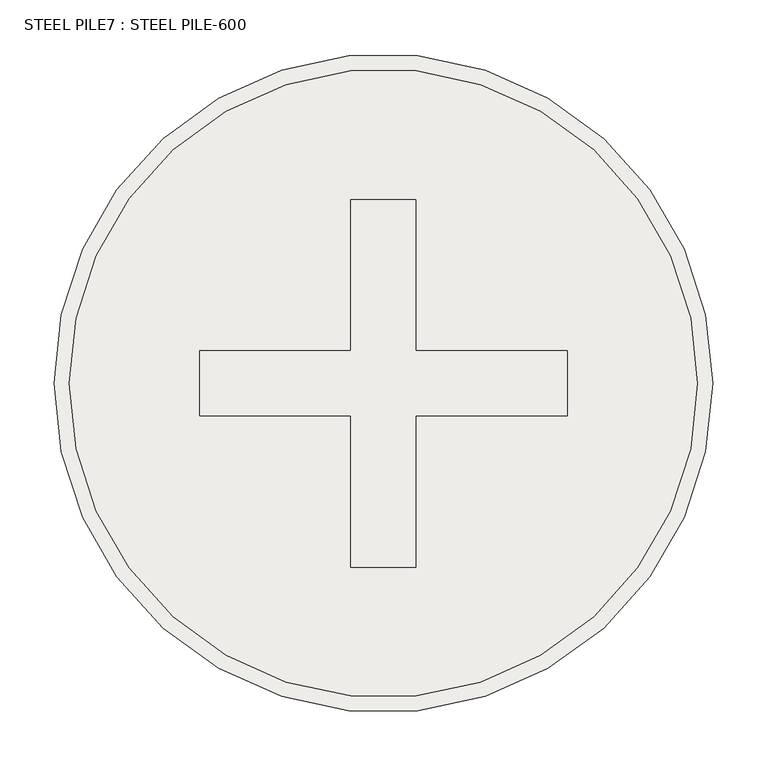
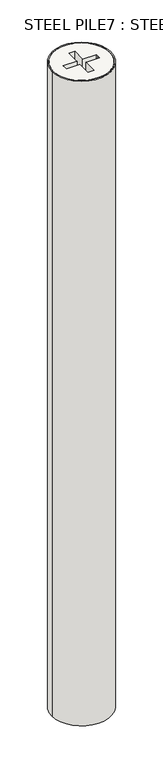
"""IFC4 building model written with IfcOpenShell, lengths in millimetres: slab geometry, STEEL PILE7 : STEEL PILE-600."""

from ifc_helpers import new_model, si_unit, point, frame, frame_2d, origin, place, context, project, spatial, circle_curve, trimmed, segment, composite_curve, outline, extrude, source, transform, mapped, element, save
from ifc_brep_helpers import plane_surface, cylinder_surface, advanced_brep


def steel_pile7_steel_pile_600_8fff8169(model_context):
    return source(origin(), model_context, "Body", "SolidModel", [
        advanced_brep(
        [(14709.5, 22499.5208589, 150.0), (15290.5, 22499.5208589, 150.0), (14970.0, 22469.5208589, 150.0), (14830.0, 22469.5208589, 150.0), (14830.0, 22499.5208589, 150.0), (14830.0, 22529.5208589, 150.0), (14970.0, 22529.5208589, 150.0), (14970.0, 22669.5208589, 150.0), (15030.0, 22669.5208589, 150.0), (15030.0, 22529.5208589, 150.0), (15170.0, 22529.5208589, 150.0), (15170.0, 22499.5208589, 150.0), (15170.0, 22469.5208589, 150.0), (15030.0, 22469.5208589, 150.0), (15030.0, 22329.5208589, 150.0), (14970.0, 22329.5208589, 150.0), (14709.5, 22499.5208589, -1850.0), (15290.5, 22499.5208589, -1850.0), (14830.0, 22469.5208589, -160.0), (14970.0, 22469.5208589, -160.0), (14970.0, 22329.5208589, -160.0), (15030.0, 22329.5208589, -160.0), (15030.0, 22469.5208589, -160.0), (15170.0, 22469.5208589, -160.0), (15170.0, 22499.5208589, -160.0), (15170.0, 22529.5208589, -160.0), (15030.0, 22529.5208589, -160.0), (15030.0, 22669.5208589, -160.0), (14970.0, 22669.5208589, -160.0), (14970.0, 22529.5208589, -160.0), (14830.0, 22529.5208589, -160.0), (14830.0, 22499.5208589, -160.0)],
        [
            (0, 1, circle_curve(frame((15000.0, 22499.5208589, 150.0), z_axis=(0.0, 0.0, 1.0), x_axis=(1.0, 0.0, 0.0)), 290.5)),
            (1, 0, circle_curve(frame((15000.0, 22499.5208589, 150.0), z_axis=(0.0, 0.0, 1.0), x_axis=(1.0, 0.0, 0.0)), 290.5)),
            (2, 3),
            (3, 4),
            (4, 5),
            (5, 6),
            (6, 7),
            (7, 8),
            (8, 9),
            (9, 10),
            (10, 11),
            (11, 12),
            (12, 13),
            (13, 14),
            (14, 15),
            (15, 2),
            (16, 17, circle_curve(frame((15000.0, 22499.5208589, -1850.0), z_axis=(0.0, 0.0, -1.0), x_axis=(1.0, 0.0, 0.0)), 290.5)),
            (17, 16, circle_curve(frame((15000.0, 22499.5208589, -1850.0), z_axis=(0.0, 0.0, -1.0), x_axis=(1.0, 0.0, 0.0)), 290.5)),
            (0, 16),
            (17, 1),
            (18, 19),
            (19, 20),
            (20, 21),
            (21, 22),
            (22, 23),
            (23, 24),
            (24, 25),
            (25, 26),
            (26, 27),
            (27, 28),
            (28, 29),
            (29, 30),
            (30, 31),
            (31, 18),
            (18, 3),
            (2, 19),
            (15, 20),
            (14, 21),
            (13, 22),
            (12, 23),
            (11, 24),
            (10, 25),
            (9, 26),
            (8, 27),
            (7, 28),
            (6, 29),
            (5, 30),
            (4, 31),
        ],
        [
            plane_surface(frame((15290.5, 22499.5208589, 150.0), z_axis=(0.0, 0.0, 1.0), x_axis=(0.0, 1.0, 0.0))),
            plane_surface(frame((15290.5, 22499.5208589, -1850.0), z_axis=(0.0, 0.0, -1.0), x_axis=(0.0, -1.0, 0.0))),
            cylinder_surface(frame((15000.0, 22499.5208589, -1850.0), z_axis=(0.0, 0.0, 1.0), x_axis=(1.0, 0.0, 0.0)), 290.5),
            plane_surface(frame((14830.0, 22469.5208589, -160.0), z_axis=(0.0, 0.0, 1.0), x_axis=(-1.0, 0.0, 0.0))),
            plane_surface(frame((14830.0, 22469.5208589, 160.0), z_axis=(0.0, 1.0, 0.0), x_axis=(0.0, 0.0, -1.0))),
            plane_surface(frame((14970.0, 22469.5208589, 160.0), z_axis=(1.0, 0.0, 0.0), x_axis=(0.0, 0.0, -1.0))),
            plane_surface(frame((14970.0, 22329.5208589, 160.0), z_axis=(0.0, 1.0, 0.0), x_axis=(0.0, 0.0, -1.0))),
            plane_surface(frame((15030.0, 22329.5208589, 160.0), z_axis=(-1.0, 0.0, 0.0), x_axis=(0.0, 0.0, -1.0))),
            plane_surface(frame((15030.0, 22469.5208589, 160.0), z_axis=(0.0, 1.0, 0.0), x_axis=(0.0, 0.0, -1.0))),
            plane_surface(frame((15170.0, 22469.5208589, 160.0), z_axis=(-1.0, 0.0, 0.0), x_axis=(0.0, 0.0, -1.0))),
            plane_surface(frame((15170.0, 22499.5208589, 160.0), z_axis=(-1.0, 0.0, 0.0), x_axis=(0.0, 0.0, -1.0))),
            plane_surface(frame((15170.0, 22529.5208589, 160.0), z_axis=(0.0, -1.0, 0.0), x_axis=(0.0, 0.0, -1.0))),
            plane_surface(frame((15030.0, 22529.5208589, 160.0), z_axis=(-1.0, 0.0, 0.0), x_axis=(0.0, 0.0, -1.0))),
            plane_surface(frame((15030.0, 22669.5208589, 160.0), z_axis=(0.0, -1.0, 0.0), x_axis=(0.0, 0.0, -1.0))),
            plane_surface(frame((14970.0, 22669.5208589, 160.0), z_axis=(1.0, 0.0, 0.0), x_axis=(0.0, 0.0, -1.0))),
            plane_surface(frame((14970.0, 22529.5208589, 160.0), z_axis=(0.0, -1.0, 0.0), x_axis=(0.0, 0.0, -1.0))),
            plane_surface(frame((14830.0, 22529.5208589, 160.0), z_axis=(1.0, 0.0, 0.0), x_axis=(0.0, 0.0, -1.0))),
            plane_surface(frame((14830.0, 22499.5208589, 160.0), z_axis=(1.0, 0.0, 0.0), x_axis=(0.0, 0.0, -1.0))),
        ],
        [
            (0, [[1, 2], [3, 4, 5, 6, 7, 8, 9, 10, 11, 12, 13, 14, 15, 16]]),
            (1, [[17, 18]]),
            (2, [[-1, 19, -18, 20]]),
            (2, [[-2, -20, -17, -19]]),
            (3, [[21, 22, 23, 24, 25, 26, 27, 28, 29, 30, 31, 32, 33, 34]]),
            (4, [[-21, 35, -3, 36]]),
            (5, [[-22, -36, -16, 37]]),
            (6, [[-23, -37, -15, 38]]),
            (7, [[-24, -38, -14, 39]]),
            (8, [[-25, -39, -13, 40]]),
            (9, [[-26, -40, -12, 41]]),
            (10, [[-27, -41, -11, 42]]),
            (11, [[-28, -42, -10, 43]]),
            (12, [[-29, -43, -9, 44]]),
            (13, [[-30, -44, -8, 45]]),
            (14, [[-31, -45, -7, 46]]),
            (15, [[-32, -46, -6, 47]]),
            (16, [[-33, -47, -5, 48]]),
            (17, [[-34, -48, -4, -35]]),
        ],
    ),
        extrude(outline(composite_curve([segment(trimmed(circle_curve(frame_2d((15000.0, 22499.5208589)), 304.5), [point((14695.5, 22499.5208589))], [point((15304.5, 22499.5208589))], False, "CARTESIAN"), True, "CONTINUOUS"), segment(trimmed(circle_curve(frame_2d((15000.0, 22499.5208589)), 304.5), [point((15304.5, 22499.5208589))], [point((14695.5, 22499.5208589))], False, "CARTESIAN"), True, "CONTINUOUS")], self_intersect=False), holes=[composite_curve([segment(trimmed(circle_curve(frame_2d((15000.0, 22499.5208589)), 290.5), [point((14709.5, 22499.5208589))], [point((15290.5, 22499.5208589))], True, "CARTESIAN"), True, "CONTINUOUS"), segment(trimmed(circle_curve(frame_2d((15000.0, 22499.5208589)), 290.5), [point((15290.5, 22499.5208589))], [point((14709.5, 22499.5208589))], True, "CARTESIAN"), True, "CONTINUOUS")], self_intersect=False)]), frame((0.0, 0.0, -6850.0), z_axis=(0.0, 0.0, 1.0), x_axis=(1.0, 0.0, 0.0)), (0.0, 0.0, 1.0), 7000.0),
    ])


if __name__ == "__main__":
    model = new_model("IFC4")
    model_context = context("Model", 3, world=origin())
    ifc_project = project(units=[si_unit("LENGTHUNIT", "METRE", prefix="MILLI")], contexts=[model_context])
    site = spatial("IfcSite", under=ifc_project)
    building = spatial("IfcBuilding", under=site)
    placement = place(None, origin())
    steel_pile7_steel_pile_600_shape = steel_pile7_steel_pile_600_8fff8169(model_context)
    element("IfcSlab", 1, ObjectType="STEEL PILE7 : STEEL PILE-600", at=placement, inside=building, context=model_context, shape_type="MappedRepresentation", body=[
        mapped(steel_pile7_steel_pile_600_shape, transform((0.0, 0.0, 0.0), x_axis=(1.0, 0.0, 0.0), y_axis=(0.0, 1.0, 0.0), z_axis=(0.0, 0.0, 1.0))),
    ])
    save(model, "model.ifc")
